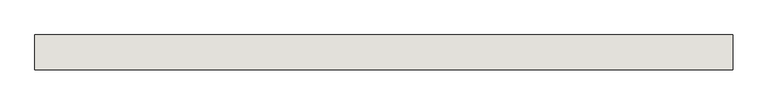
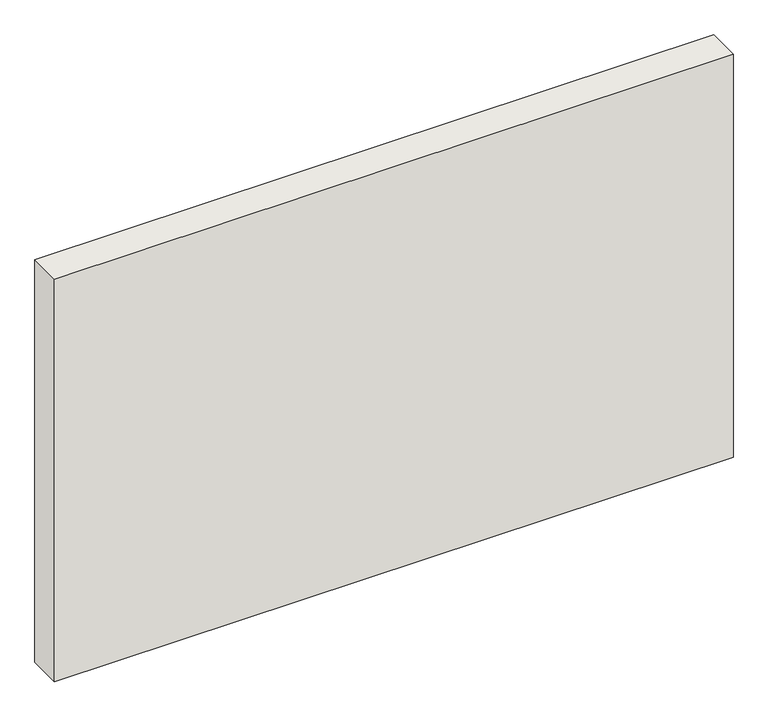
"""IFC4 building model written with IfcOpenShell, lengths in millimetres: wall geometry, Holzwand."""

from ifc_helpers import new_model, si_unit, origin, origin_with_axes, place, context, project, spatial, polyline, outline, extrude, source, transform, mapped, element, save


def wall_219f7194(model_context):
    return source(origin(), model_context, "Body", "SweptSolid", [
        extrude(outline(polyline([(0.0, 200.0), (4000.0, 200.0), (4000.0, 0.0), (0.0, 0.0), (0.0, 200.0)])), origin_with_axes(), (0.0, 0.0, 1.0), 2510.0),
    ])


if __name__ == "__main__":
    model = new_model("IFC4")
    model_context = context("Model", 3, world=origin())
    ifc_project = project(units=[si_unit("LENGTHUNIT", "METRE", prefix="MILLI")], contexts=[model_context])
    site = spatial("IfcSite", under=ifc_project)
    building = spatial("IfcBuilding", under=site)
    placement = place(None, origin())
    wall_shape = wall_219f7194(model_context)
    element("IfcWall", 1, ObjectType="Holzwand", at=placement, inside=building, context=model_context, shape_type="MappedRepresentation", body=[
        mapped(wall_shape, transform((0.0, 0.0, 0.0), x_axis=(1.0, 0.0, 0.0), y_axis=(0.0, 1.0, 0.0), z_axis=(0.0, 0.0, 1.0))),
    ])
    save(model, "model.ifc")

# Revit data of these elements
# Element 1 (IfcWall, "Holzwand")
#   Materials on its faces: "holzschalung"
# Materials
#   "holzschalung": class "Unassigned", colour RGB 128 128 128, transparency 0
